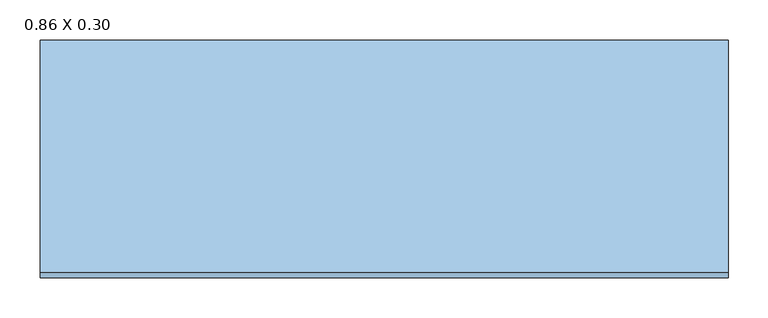
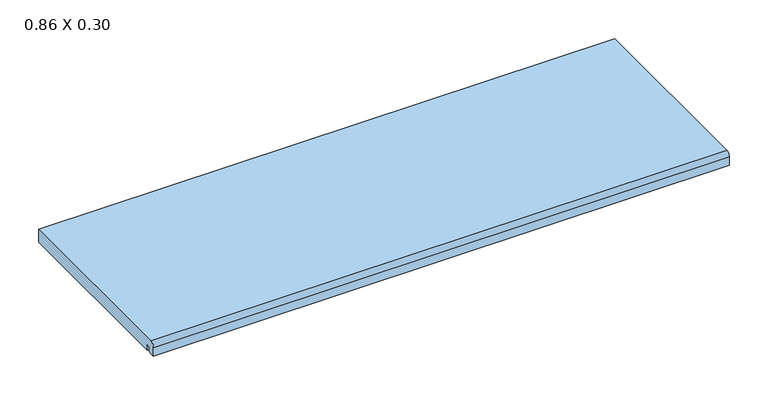
"""IFC4 building model written with IfcOpenShell, lengths in millimetres: window geometry, .CC_ND 300_PEDRA_PEITORIL RETO : 0.86 X 0.30."""

from ifc_helpers import new_model, si_unit, point, frame, frame_2d, origin, place, context, project, spatial, polyline, circle_curve, trimmed, segment, composite_curve, outline, extrude, source, transform, mapped, element, save


def window_0_86_x_0_30_a250a5e5(model_context):
    return source(origin(), model_context, "Body", "SweptSolid", [
        extrude(outline(composite_curve([segment(polyline([(-132.5083081, 1480.0), (-132.5083081, 1488.1993124), (-137.2619526, 1488.1993124), (-137.2619526, 1480.0), (-148.0, 1480.0), (-148.0, 1493.3808343)]), True, "CONTINUOUS"), segment(trimmed(circle_curve(frame_2d((-141.3808343, 1493.3808343)), 6.6191657), [point((-148.0, 1493.3808343))], [point((-141.3808343, 1500.0))], False, "CARTESIAN"), True, "CONTINUOUS"), segment(polyline([(-141.3808343, 1500.0), (149.0, 1500.0), (149.0, 1480.0), (-132.5083081, 1480.0)]), True, "CONTINUOUS")], self_intersect=False)), frame((-430.0, 0.0, 0.0), z_axis=(1.0, 0.0, 0.0), x_axis=(0.0, 1.0, 0.0)), (0.0, 0.0, 1.0), 860.0),
    ])


if __name__ == "__main__":
    model = new_model("IFC4")
    model_context = context("Model", 3, world=origin())
    ifc_project = project(units=[si_unit("LENGTHUNIT", "METRE", prefix="MILLI")], contexts=[model_context])
    site = spatial("IfcSite", under=ifc_project)
    building = spatial("IfcBuilding", under=site)
    placement = place(None, origin())
    window_0_86_x_0_30_shape = window_0_86_x_0_30_a250a5e5(model_context)
    element("IfcWindow", 1, ObjectType=".CC_ND 300_PEDRA_PEITORIL RETO : 0.86 X 0.30", at=placement, inside=building, context=model_context, shape_type="MappedRepresentation", body=[
        mapped(window_0_86_x_0_30_shape, transform((0.0, 0.0, 0.0), x_axis=(1.0, 0.0, 0.0), y_axis=(0.0, 1.0, 0.0), z_axis=(0.0, 0.0, 1.0))),
    ])
    save(model, "model.ifc")

# Revit data of these elements
# Type ".CC_ND 300_PEDRA_PEITORIL RETO : 0.86 X 0.30"
#   Type Mark = "66"
#   Largura da pedra [instance default] = 0.26 m
#   Extensão interior peitoril [instance default] = 0.03 m
#   Extensão exterior peitoril [instance default] = 0.03 m
#   Espessura = 0.02 m
#   Comprimento = 0.86 m
#   Altura-padrão do peitoril = 1.48 m
#   Peitoril = .GRANITO_BRANCO_ITAUNAS
#   Rough Width = 0
#   Rough Height = 0
#   Height = 0
#   Wall Closure = (empty or 0)
#   Width = 0
# Element 1 (IfcWindow, ".CC_ND 300_PEDRA_PEITORIL RETO : 0.86 X 0.30")
#   Largura da pedra = 0.297 m
#   Extensão interior peitoril = 0.031 m
#   Materials on its faces: ".GRANITO_BRANCO_ITAUNAS"
# Materials
#   ".GRANITO_BRANCO_ITAUNAS": class ".CC_PEDRA REVEST.", colour RGB 202 195 174, transparency 0, Description = "Revestimento em granito", Cost = 0
